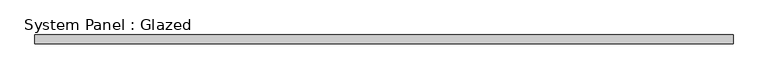
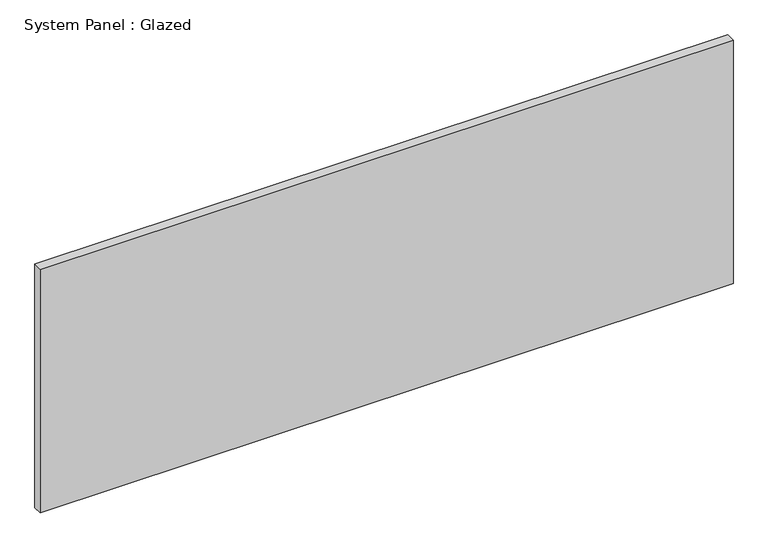
"""IFC4 building model written with IfcOpenShell, lengths in millimetres: plate geometry, System Panel : Glazed."""

from ifc_helpers import new_model, si_unit, origin, origin_with_axes, place, context, project, spatial, polyline, outline, extrude, source, transform, mapped, element, save


def system_panel_glazed_bc1ebc0c(model_context):
    return source(origin(), model_context, "Body", "SweptSolid", [
        extrude(outline(polyline([(975.0000002, 24.5), (-975.0000002, 24.5), (-975.0000002, 49.5), (975.0000002, 49.5), (975.0000002, 24.5)])), origin_with_axes(), (0.0, 0.0, 1.0), 725.0),
    ])


if __name__ == "__main__":
    model = new_model("IFC4")
    model_context = context("Model", 3, world=origin())
    ifc_project = project(units=[si_unit("LENGTHUNIT", "METRE", prefix="MILLI")], contexts=[model_context])
    site = spatial("IfcSite", under=ifc_project)
    building = spatial("IfcBuilding", under=site)
    placement = place(None, origin())
    system_panel_glazed_shape = system_panel_glazed_bc1ebc0c(model_context)
    element("IfcPlate", 1, ObjectType="System Panel : Glazed", at=placement, inside=building, context=model_context, shape_type="MappedRepresentation", body=[
        mapped(system_panel_glazed_shape, transform((0.0, 0.0, 0.0), x_axis=(1.0, 0.0, 0.0), y_axis=(0.0, 1.0, 0.0), z_axis=(0.0, 0.0, 1.0))),
    ])
    save(model, "model.ifc")

# Revit data of these elements
# Element 1 (IfcPlate, "System Panel : Glazed")
#   Materials on its faces: "Glass"
# Materials
#   "Glass": class "Glass", colour RGB 0 128 192, transparency 0.9
